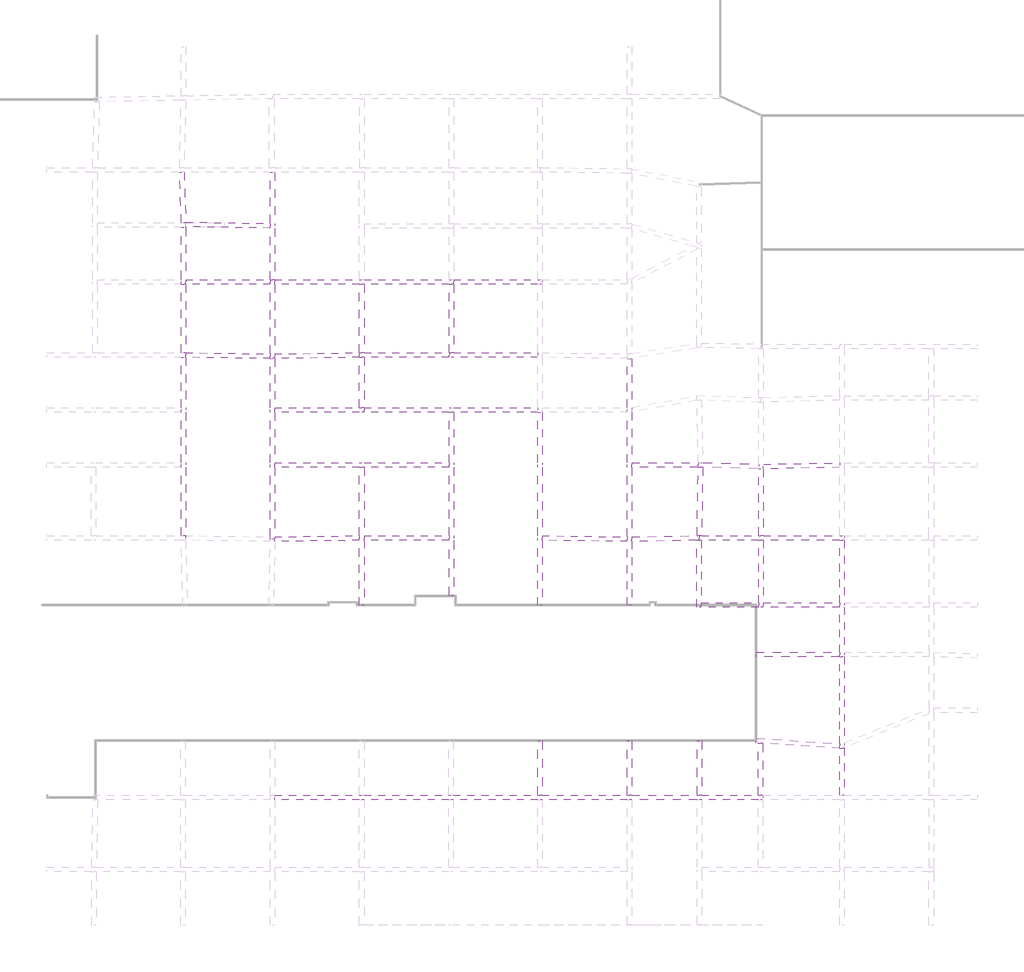
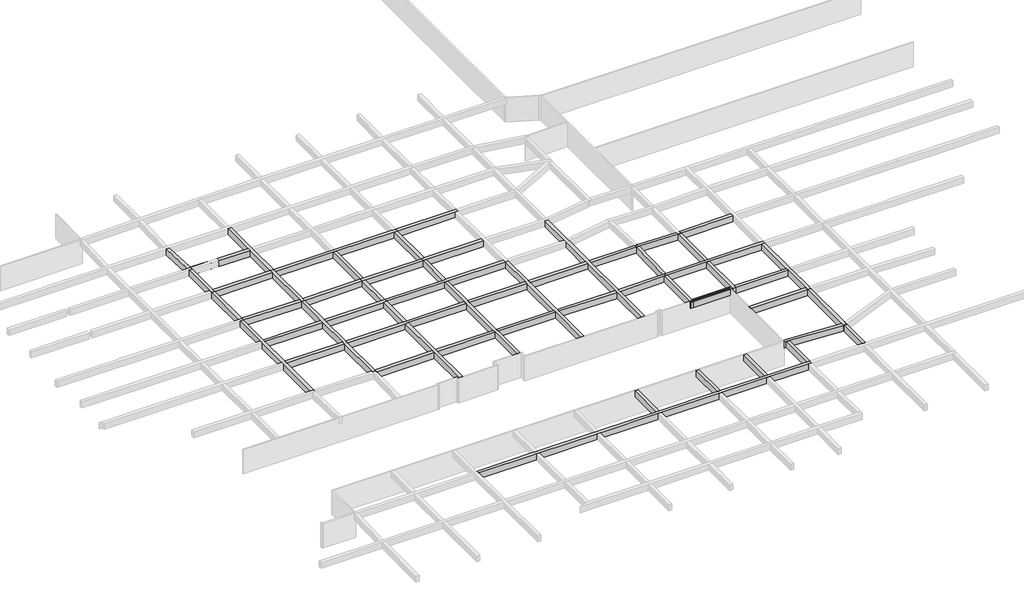
# One storey, part 14 of 20: 49 beams.
"""IFC4 building model written with IfcOpenShell, lengths in millimetres."""

from ifc_helpers import new_model, si_unit, frame, origin, place, context, project, spatial, polyline, outline, extrude, faceted_brep, element, save

model = new_model("IFC4")

# Units and contexts
model_context = context("Model", 3, world=origin())
ifc_project = project(units=[si_unit("LENGTHUNIT", "METRE", prefix="MILLI")], contexts=[model_context])

# Site, building, storey
site = spatial("IfcSite", under=ifc_project)
building = spatial("IfcBuilding", under=site)
storey = spatial("IfcBuildingStorey", under=building, Name="户型图", Elevation=0.0)

# Beams
placement = place(None, origin())
element("IfcBeam", 1, ObjectType="混凝土 - 矩形梁 : KL_beam", at=placement, inside=storey, context=model_context, shape_type="Brep", body=[
    faceted_brep([(183030.0, 66190.0, 3300.0), (183030.0, 66590.0, 3300.0), (182630.0, 66590.0, 3300.0), (177676.0, 66590.0, 3300.0), (177276.0, 66590.0, 3300.0), (171550.0, 66590.0, 3300.0), (171150.0, 66590.0, 3300.0), (163750.0, 66590.0, 3300.0), (163350.0, 66590.0, 3300.0), (155950.0, 66590.0, 3300.0), (155550.0, 66590.0, 3300.0), (148150.0, 66590.0, 3300.0), (147750.0, 66590.0, 3300.0), (140350.0, 66590.0, 3300.0), (140350.0, 66190.0, 3300.0), (147750.0, 66190.0, 3300.0), (148150.0, 66190.0, 3300.0), (155550.0, 66190.0, 3300.0), (155950.0, 66190.0, 3300.0), (163350.0, 66190.0, 3300.0), (163750.0, 66190.0, 3300.0), (171150.0, 66190.0, 3300.0), (171550.0, 66190.0, 3300.0), (177276.0, 66190.0, 3300.0), (177676.0, 66190.0, 3300.0), (182630.0, 66190.0, 3300.0), (183030.0, 66190.0, 2500.0), (140350.0, 66190.0, 2500.0), (147750.0, 66190.0, 2500.0), (148150.0, 66190.0, 2500.0), (155550.0, 66190.0, 2500.0), (155950.0, 66190.0, 2500.0), (163350.0, 66190.0, 2500.0), (163750.0, 66190.0, 2500.0), (171150.0, 66190.0, 2500.0), (171550.0, 66190.0, 2500.0), (177276.0, 66190.0, 2500.0), (177676.0, 66190.0, 2500.0), (182630.0, 66190.0, 2500.0), (183030.0, 66590.0, 2500.0), (140350.0, 66590.0, 2500.0), (147750.0, 66590.0, 2500.0), (148150.0, 66590.0, 2500.0), (155550.0, 66590.0, 2500.0), (155950.0, 66590.0, 2500.0), (163350.0, 66590.0, 2500.0), (163750.0, 66590.0, 2500.0), (171150.0, 66590.0, 2500.0), (171550.0, 66590.0, 2500.0), (177276.0, 66590.0, 2500.0), (177676.0, 66590.0, 2500.0), (182630.0, 66590.0, 2500.0)], [[[0, 1, 2, 3, 4, 5, 6, 7, 8, 9, 10, 11, 12, 13, 14, 15, 16, 17, 18, 19, 20, 21, 22, 23, 24, 25]], [[26, 0, 25, 24, 23, 22, 21, 20, 19, 18, 17, 16, 15, 14, 27, 28, 29, 30, 31, 32, 33, 34, 35, 36, 37, 38]], [[39, 26, 38, 37, 36, 35, 34, 33, 32, 31, 30, 29, 28, 27, 40, 41, 42, 43, 44, 45, 46, 47, 48, 49, 50, 51]], [[1, 39, 51, 50, 49, 48, 47, 46, 45, 44, 43, 42, 41, 40, 13, 12, 11, 10, 9, 8, 7, 6, 5, 4, 3, 2]], [[14, 13, 40, 27]], [[1, 0, 26, 39]]]),
])
element("IfcBeam", 2, ObjectType="混凝土 - 矩形梁 : KL_beam", at=placement, inside=storey, context=model_context, shape_type="Brep", body=[
    faceted_brep([(132150.0, 89290.0, 3300.0), (132544.9959727, 89290.0, 3300.0), (132550.0, 89092.5337107, 3300.0), (132550.0, 89287.4523333, 3300.0), (132550.0, 95290.0, 3300.0), (132550.0, 95690.0, 3300.0), (132550.0, 100089.0, 3300.0), (132550.0, 100489.0, 3300.0), (132550.0, 104885.6852836, 3300.0), (132550.0, 104889.0, 3300.0), (132150.0, 104889.0, 3300.0), (132150.0, 100489.0, 3300.0), (132150.0, 100089.0, 3300.0), (132150.0, 95690.0, 3300.0), (132150.0, 95290.0, 3300.0), (132150.0, 89290.0, 2500.0), (132150.0, 104889.0, 2500.0), (132150.0, 100489.0, 2500.0), (132150.0, 100089.0, 2500.0), (132150.0, 95690.0, 2500.0), (132150.0, 95290.0, 2500.0), (132544.9959727, 89290.0, 2500.0), (132550.0, 104889.0, 2500.0), (132550.0, 104885.6852836, 2500.0), (132550.0, 100489.0, 2500.0), (132550.0, 100089.0, 2500.0), (132550.0, 95690.0, 2500.0), (132550.0, 95290.0, 2500.0), (132550.0, 89287.4523333, 2500.0), (132550.0, 89092.5337107, 2500.0)], [[[0, 1, 2, 3, 4, 5, 6, 7, 8, 9, 10, 11, 12, 13, 14]], [[15, 0, 14, 13, 12, 11, 10, 16, 17, 18, 19, 20]], [[21, 15, 20, 19, 18, 17, 16, 22, 23, 24, 25, 26, 27, 28, 29]], [[2, 29, 28, 27, 26, 25, 24, 23, 22, 9, 8, 7, 6, 5, 4, 3]], [[21, 1, 0, 15]], [[1, 21, 29, 2]], [[10, 9, 22, 16]]]),
])
element("IfcBeam", 3, ObjectType="混凝土 - 矩形梁 : KL_beam", at=placement, inside=storey, context=model_context, shape_type="Brep", body=[
    faceted_brep([(132412.7389969, 121089.0, 3300.0), (132012.4951791, 121089.0, 3300.0), (132167.2640295, 116657.0, 3300.0), (132567.5078472, 116657.0, 3300.0), (132565.6031542, 116711.5432728, 3300.0), (132012.4951791, 121089.0, 2500.0), (132167.2640295, 116657.0, 2500.0), (132412.7389969, 121089.0, 2500.0), (132565.6031542, 116711.5432728, 2500.0), (132567.5078472, 116657.0, 2500.0)], [[[0, 1, 2, 3, 4]], [[1, 5, 6, 2]], [[5, 7, 8, 9, 6]], [[7, 0, 4, 3, 9, 8]], [[1, 0, 7, 5]], [[3, 2, 6, 9]]]),
])
element("IfcBeam", 4, ObjectType="混凝土 - 矩形梁 : KL_beam", at=placement, inside=storey, context=model_context, shape_type="Brep", body=[
    faceted_brep([(132172.3572995, 111289.0, 2500.0), (132172.3572995, 111289.0, 3300.0), (132172.3572995, 111689.0, 3300.0), (132172.3572995, 116257.0, 3300.0), (132172.3572995, 116257.0, 2500.0), (132172.3572995, 111689.0, 2500.0), (132572.3572995, 111289.0, 3300.0), (132572.3572995, 111289.0, 2500.0), (132572.3572995, 116257.0, 3300.0), (132572.3572995, 116257.0, 2500.0), (132572.3572995, 111689.0, 3300.0), (132572.3572995, 111689.0, 2500.0)], [[[0, 1, 2, 3, 4, 5]], [[6, 1, 0, 7]], [[8, 9, 4, 3]], [[1, 6, 10, 8, 3, 2]], [[7, 0, 5, 4, 9, 11]], [[6, 7, 11, 9, 8, 10]]]),
])
element("IfcBeam", 5, ObjectType="混凝土 - 矩形梁 : KL_beam", at=placement, inside=storey, context=model_context, shape_type="Brep", body=[
    faceted_brep([(132550.0, 104889.0, 3300.0), (132572.3572995, 104889.0, 3300.0), (132572.3572995, 105285.4331901, 3300.0), (132572.3572995, 111289.0, 3300.0), (132172.3572995, 111289.0, 3300.0), (132172.3572995, 105289.0, 3300.0), (132550.0, 105289.0, 3300.0), (132172.3572995, 105289.0, 2500.0), (132172.3572995, 111289.0, 2500.0), (132572.3572995, 104889.0, 2500.0), (132550.0, 104889.0, 2500.0), (132550.0, 105289.0, 2500.0), (132572.3572995, 111289.0, 2500.0), (132572.3572995, 105285.4331901, 2500.0)], [[[0, 1, 2, 3, 4, 5, 6]], [[7, 5, 4, 8]], [[9, 10, 11, 7, 8, 12, 13]], [[1, 9, 13, 12, 3, 2]], [[9, 1, 0, 10]], [[11, 6, 5, 7]], [[6, 11, 10, 0]], [[4, 3, 12, 8]]]),
])
element("IfcBeam", 6, ObjectType="混凝土 - 矩形梁 : KL_beam", at=placement, inside=storey, context=model_context, shape_type="Brep", body=[
    faceted_brep([(139950.0, 104791.5476667, 3300.0), (140350.0, 104791.5476667, 3300.0), (140350.0, 105191.5805384, 3300.0), (140350.0, 111289.0, 3300.0), (140350.0, 111689.0, 3300.0), (139950.0, 111689.0, 3300.0), (139950.0, 111289.0, 3300.0), (139950.0, 105191.5609646, 3300.0), (140350.0, 104791.5476667, 2500.0), (140350.0, 105191.5805384, 2500.0), (140350.0, 111289.0, 2500.0), (140350.0, 111689.0, 2500.0), (139950.0, 104791.5476667, 2500.0), (139950.0, 105191.5609646, 2500.0), (139950.0, 111289.0, 2500.0), (139950.0, 111689.0, 2500.0)], [[[0, 1, 2, 3, 4, 5, 6, 7]], [[1, 8, 9, 10, 11, 4, 3, 2]], [[8, 12, 13, 14, 15, 11, 10, 9]], [[12, 0, 7, 6, 5, 15, 14, 13]], [[5, 4, 11, 15]], [[0, 12, 8, 1]]]),
])
element("IfcBeam", 7, ObjectType="混凝土 - 矩形梁 : KL_beam", at=placement, inside=storey, context=model_context, shape_type="SweptSolid", body=[
    extrude(outline(polyline([(132572.3572995, 111289.0), (132572.3572995, 111689.0), (139950.0, 111689.0), (139950.0, 111289.0), (132572.3572995, 111289.0)])), frame((0.0, 0.0, 2500.0), z_axis=(0.0, 0.0, 1.0), x_axis=(1.0, 0.0, 0.0)), (0.0, 0.0, 1.0), 800.0),
])
element("IfcBeam", 8, ObjectType="混凝土 - 矩形梁 : KL_beam", at=placement, inside=storey, context=model_context, shape_type="Brep", body=[
    faceted_brep([(139950.0, 111689.0, 3300.0), (140350.0, 111689.0, 3300.0), (140350.0, 116189.0, 3300.0), (140350.0, 116589.0, 3300.0), (140350.0, 121089.0, 3300.0), (139950.0, 121089.0, 3300.0), (139950.0, 116592.2568622, 3300.0), (139950.0, 116192.2046763, 3300.0), (140350.0, 111689.0, 2500.0), (140350.0, 116189.0, 2500.0), (140350.0, 116589.0, 2500.0), (140350.0, 121089.0, 2500.0), (139950.0, 111689.0, 2500.0), (139950.0, 116192.2046763, 2500.0), (139950.0, 116592.2568622, 2500.0), (139950.0, 121089.0, 2500.0)], [[[0, 1, 2, 3, 4, 5, 6, 7]], [[1, 8, 9, 10, 11, 4, 3, 2]], [[8, 12, 13, 14, 15, 11, 10, 9]], [[12, 0, 7, 6, 5, 15, 14, 13]], [[1, 0, 12, 8]], [[5, 4, 11, 15]]]),
])
element("IfcBeam", 9, ObjectType="混凝土 - 矩形梁 : KL_beam", at=placement, inside=storey, context=model_context, shape_type="SweptSolid", body=[
    extrude(outline(polyline([(132572.3572995, 116518.1298566), (132572.3572995, 116657.0), (132567.5078472, 116657.0), (132565.6031542, 116711.5432728), (139950.0, 116592.2568622), (139950.0, 116192.2046763), (132579.5811694, 116311.2652881), (132572.3572995, 116518.1298566)])), frame((0.0, 0.0, 2500.0), z_axis=(0.0, 0.0, 1.0), x_axis=(1.0, 0.0, 0.0)), (0.0, 0.0, 1.0), 800.0),
])
element("IfcBeam", 10, ObjectType="混凝土 - 矩形梁 : KL_beam", at=placement, inside=storey, context=model_context, shape_type="Brep", body=[
    faceted_brep([(155979.0, 111289.0, 3300.0), (155979.0, 111689.0, 3300.0), (155579.0, 111689.0, 3300.0), (148150.0, 111689.0, 3300.0), (147750.0, 111689.0, 3300.0), (140350.0, 111689.0, 3300.0), (140350.0, 111289.0, 3300.0), (147750.0, 111289.0, 3300.0), (148150.0, 111289.0, 3300.0), (155579.0, 111289.0, 3300.0), (155979.0, 111289.0, 2500.0), (140350.0, 111289.0, 2500.0), (147750.0, 111289.0, 2500.0), (148150.0, 111289.0, 2500.0), (155579.0, 111289.0, 2500.0), (155979.0, 111689.0, 2500.0), (140350.0, 111689.0, 2500.0), (147750.0, 111689.0, 2500.0), (148150.0, 111689.0, 2500.0), (155579.0, 111689.0, 2500.0)], [[[0, 1, 2, 3, 4, 5, 6, 7, 8, 9]], [[10, 0, 9, 8, 7, 6, 11, 12, 13, 14]], [[15, 10, 14, 13, 12, 11, 16, 17, 18, 19]], [[1, 15, 19, 18, 17, 16, 5, 4, 3, 2]], [[6, 5, 16, 11]], [[1, 0, 10, 15]]]),
])
element("IfcBeam", 11, ObjectType="混凝土 - 矩形梁 : KL_beam", at=placement, inside=storey, context=model_context, shape_type="Brep", body=[
    faceted_brep([(163750.0, 111289.0, 3300.0), (163750.0, 111689.0, 3300.0), (163350.0, 111689.0, 3300.0), (155979.0, 111689.0, 3300.0), (155979.0, 111289.0, 3300.0), (163350.0, 111289.0, 3300.0), (163750.0, 111289.0, 2500.0), (155979.0, 111289.0, 2500.0), (163350.0, 111289.0, 2500.0), (163750.0, 111689.0, 2500.0), (155979.0, 111689.0, 2500.0), (163350.0, 111689.0, 2500.0)], [[[0, 1, 2, 3, 4, 5]], [[6, 0, 5, 4, 7, 8]], [[9, 6, 8, 7, 10, 11]], [[1, 9, 11, 10, 3, 2]], [[4, 3, 10, 7]], [[1, 0, 6, 9]]]),
])
element("IfcBeam", 12, ObjectType="混凝土 - 矩形梁 : KL_beam", at=placement, inside=storey, context=model_context, shape_type="Brep", body=[
    faceted_brep([(155579.0, 104889.0, 3300.0), (155579.0, 104889.0, 2500.0), (155979.0, 104889.0, 2500.0), (163350.0, 104889.0, 2500.0), (163350.0, 104889.0, 3300.0), (155979.0, 104889.0, 3300.0), (155579.0, 105289.0, 3300.0), (155579.0, 105289.0, 2500.0), (163350.0, 105289.0, 2500.0), (163350.0, 105289.0, 3300.0), (155979.0, 105289.0, 3300.0), (155979.0, 105289.0, 2500.0)], [[[0, 1, 2, 3, 4, 5]], [[0, 6, 7, 1]], [[4, 3, 8, 9]], [[6, 0, 5, 4, 9, 10]], [[7, 6, 10, 9, 8, 11]], [[1, 7, 11, 8, 3, 2]]]),
])
element("IfcBeam", 13, ObjectType="混凝土 - 矩形梁 : KL_beam", at=placement, inside=storey, context=model_context, shape_type="Brep", body=[
    faceted_brep([(147750.0, 105289.0, 3300.0), (147750.0, 105286.4523333, 3300.0), (147750.0, 104889.0, 3300.0), (148150.0, 104889.0, 3300.0), (155579.0, 104889.0, 3300.0), (155579.0, 105289.0, 3300.0), (148150.0, 105289.0, 3300.0), (147750.0, 105289.0, 2500.0), (155579.0, 105289.0, 2500.0), (148150.0, 105289.0, 2500.0), (147750.0, 104889.0, 2500.0), (147750.0, 105286.4523333, 2500.0), (155579.0, 104889.0, 2500.0), (148150.0, 104889.0, 2500.0)], [[[0, 1, 2, 3, 4, 5, 6]], [[7, 0, 6, 5, 8, 9]], [[10, 11, 7, 9, 8, 12, 13]], [[2, 10, 13, 12, 4, 3]], [[2, 1, 0, 7, 11, 10]], [[5, 4, 12, 8]]]),
])
element("IfcBeam", 14, ObjectType="混凝土 - 矩形梁 : KL_beam", at=placement, inside=storey, context=model_context, shape_type="SweptSolid", body=[
    extrude(outline(polyline([(148150.0, 105289.0), (147750.0, 105289.0), (147750.0, 111289.0), (148150.0, 111289.0), (148150.0, 105289.0)])), frame((0.0, 0.0, 2500.0), z_axis=(0.0, 0.0, 1.0), x_axis=(1.0, 0.0, 0.0)), (0.0, 0.0, 1.0), 800.0),
])
element("IfcBeam", 15, ObjectType="混凝土 - 矩形梁 : KL_beam", at=placement, inside=storey, context=model_context, shape_type="SweptSolid", body=[
    extrude(outline(polyline([(155579.0, 111289.0), (155979.0, 111289.0), (155979.0, 105289.0), (155579.0, 105289.0), (155579.0, 111289.0)])), frame((0.0, 0.0, 2500.0), z_axis=(0.0, 0.0, 1.0), x_axis=(1.0, 0.0, 0.0)), (0.0, 0.0, 1.0), 800.0),
])
element("IfcBeam", 16, ObjectType="混凝土 - 矩形梁 : KL_beam", at=placement, inside=storey, context=model_context, shape_type="Brep", body=[
    faceted_brep([(139950.0, 88991.7453736, 3300.0), (140350.0, 88988.2546264, 3300.0), (140350.0, 89187.4523333, 3300.0), (140350.0, 95290.0, 3300.0), (140350.0, 95690.0, 3300.0), (140350.0, 100089.0, 3300.0), (140350.0, 100489.0, 3300.0), (140350.0, 104791.5476667, 3300.0), (139950.0, 104786.4194616, 3300.0), (139950.0, 100489.0, 3300.0), (139950.0, 100089.0, 3300.0), (139950.0, 95690.0, 3300.0), (139950.0, 95290.0, 3300.0), (139950.0, 89192.5805384, 3300.0), (139950.0, 88991.7453736, 2500.0), (139950.0, 104786.4194616, 2500.0), (139950.0, 100489.0, 2500.0), (139950.0, 100089.0, 2500.0), (139950.0, 95690.0, 2500.0), (139950.0, 95290.0, 2500.0), (139950.0, 89192.5805384, 2500.0), (140350.0, 88988.2546264, 2500.0), (140350.0, 104791.5476667, 2500.0), (140350.0, 100489.0, 2500.0), (140350.0, 100089.0, 2500.0), (140350.0, 95690.0, 2500.0), (140350.0, 95290.0, 2500.0), (140350.0, 89187.4523333, 2500.0)], [[[0, 1, 2, 3, 4, 5, 6, 7, 8, 9, 10, 11, 12, 13]], [[14, 0, 13, 12, 11, 10, 9, 8, 15, 16, 17, 18, 19, 20]], [[21, 14, 20, 19, 18, 17, 16, 15, 22, 23, 24, 25, 26, 27]], [[1, 21, 27, 26, 25, 24, 23, 22, 7, 6, 5, 4, 3, 2]], [[1, 0, 14, 21]], [[8, 7, 22, 15]]]),
])
element("IfcBeam", 17, ObjectType="混凝土 - 矩形梁 : KL_beam", at=placement, inside=storey, context=model_context, shape_type="Brep", body=[
    faceted_brep([(140350.0, 88988.2546264, 3300.0), (140346.5831577, 88792.503861, 3300.0), (147750.0, 88887.4194616, 3300.0), (147750.0, 89287.4523333, 3300.0), (140350.0, 89192.5805384, 3300.0), (140350.0, 89187.4523333, 3300.0), (140346.5831577, 88792.503861, 2500.0), (147750.0, 88887.4194616, 2500.0), (140350.0, 88988.2546264, 2500.0), (140350.0, 89187.4523333, 2500.0), (140350.0, 89192.5805384, 2500.0), (147750.0, 89287.4523333, 2500.0)], [[[0, 1, 2, 3, 4, 5]], [[1, 6, 7, 2]], [[6, 8, 9, 10, 11, 7]], [[10, 4, 3, 11]], [[4, 10, 9, 8, 0, 5]], [[1, 0, 8, 6]], [[3, 2, 7, 11]]]),
])
element("IfcBeam", 18, ObjectType="混凝土 - 矩形梁 : KL_beam", at=placement, inside=storey, context=model_context, shape_type="Brep", body=[
    faceted_brep([(132550.0, 100489.0, 3300.0), (132550.0, 100089.0, 3300.0), (139950.0, 100089.0, 3300.0), (139950.0, 100489.0, 3300.0), (132550.0, 100089.0, 2500.0), (139950.0, 100089.0, 2500.0), (132550.0, 100489.0, 2500.0), (139950.0, 100489.0, 2500.0)], [[[0, 1, 2, 3]], [[1, 4, 5, 2]], [[4, 6, 7, 5]], [[6, 0, 3, 7]], [[1, 0, 6, 4]], [[3, 2, 5, 7]]]),
    faceted_brep([(140350.0, 100089.0, 3300.0), (140350.0, 100489.0, 3300.0), (140350.0, 100489.0, 2500.0), (140350.0, 100089.0, 2500.0), (148150.0, 100089.0, 3300.0), (148150.0, 100489.0, 3300.0), (147750.0, 100489.0, 3300.0), (147750.0, 100089.0, 3300.0), (148150.0, 100089.0, 2500.0), (147750.0, 100089.0, 2500.0), (148150.0, 100489.0, 2500.0), (147750.0, 100489.0, 2500.0)], [[[0, 1, 2, 3]], [[4, 5, 6, 1, 0, 7]], [[8, 4, 7, 0, 3, 9]], [[10, 8, 9, 3, 2, 11]], [[5, 10, 11, 2, 1, 6]], [[5, 4, 8, 10]]]),
])
element("IfcBeam", 19, ObjectType="混凝土 - 矩形梁 : KL_beam", at=placement, inside=storey, context=model_context, shape_type="Brep", body=[
    faceted_brep([(148150.0, 104889.0, 3300.0), (147750.0, 104889.0, 3300.0), (147750.0, 104886.4194616, 3300.0), (147750.0, 100489.0, 3300.0), (148150.0, 100489.0, 3300.0), (148150.0, 104889.0, 2500.0), (148150.0, 100489.0, 2500.0), (147750.0, 104889.0, 2500.0), (147750.0, 100489.0, 2500.0), (147750.0, 104886.4194616, 2500.0)], [[[0, 1, 2, 3, 4]], [[5, 0, 4, 6]], [[7, 5, 6, 8, 9]], [[1, 7, 9, 8, 3, 2]], [[1, 0, 5, 7]], [[4, 3, 8, 6]]]),
])
element("IfcBeam", 20, ObjectType="混凝土 - 矩形梁 : KL_beam", at=placement, inside=storey, context=model_context, shape_type="Brep", body=[
    faceted_brep([(139950.0, 104786.4194616, 3300.0), (139950.0, 104786.4194616, 2500.0), (140350.0, 104791.5476667, 2500.0), (147750.0, 104886.4194616, 2500.0), (147750.0, 104886.4194616, 3300.0), (140350.0, 104791.5476667, 3300.0), (139950.0, 104791.5476667, 3300.0), (139950.0, 104791.5476667, 2500.0), (140350.0, 105191.5805384, 3300.0), (140350.0, 105191.5805384, 2500.0), (147750.0, 104889.0, 2500.0), (147750.0, 105286.4523333, 2500.0), (147750.0, 105286.4523333, 3300.0), (147750.0, 104889.0, 3300.0)], [[[0, 1, 2, 3, 4, 5]], [[1, 0, 6, 7]], [[2, 5, 8, 9]], [[5, 2, 7, 6]], [[6, 0, 5]], [[1, 7, 2]], [[4, 3, 10, 11, 12, 13]], [[8, 5, 4, 13, 12]], [[9, 8, 12, 11]], [[2, 9, 11, 10, 3]]]),
])
element("IfcBeam", 21, ObjectType="混凝土 - 矩形梁 : KL_beam", at=placement, inside=storey, context=model_context, shape_type="SweptSolid", body=[
    extrude(outline(polyline([(139950.0, 105191.5609646), (139950.0, 104791.5285865), (132550.0, 104885.6852836), (132550.0, 104889.0), (132572.3572995, 104889.0), (132572.3572995, 105285.4331901), (139950.0, 105191.5609646)])), frame((0.0, 0.0, 2500.0), z_axis=(0.0, 0.0, 1.0), x_axis=(1.0, 0.0, 0.0)), (0.0, 0.0, 1.0), 800.0),
])
element("IfcBeam", 22, ObjectType="混凝土 - 矩形梁 : KL_beam", at=placement, inside=storey, context=model_context, shape_type="Brep", body=[
    faceted_brep([(163350.0, 100089.0, 3300.0), (163350.0, 100489.0, 3300.0), (155979.0, 100489.0, 3300.0), (155579.0, 100489.0, 3300.0), (148150.0, 100489.0, 3300.0), (148150.0, 100089.0, 3300.0), (155579.0, 100089.0, 3300.0), (155979.0, 100089.0, 3300.0), (163350.0, 100089.0, 2500.0), (148150.0, 100089.0, 2500.0), (155579.0, 100089.0, 2500.0), (155979.0, 100089.0, 2500.0), (163350.0, 100489.0, 2500.0), (148150.0, 100489.0, 2500.0), (155579.0, 100489.0, 2500.0), (155979.0, 100489.0, 2500.0)], [[[0, 1, 2, 3, 4, 5, 6, 7]], [[8, 0, 7, 6, 5, 9, 10, 11]], [[12, 8, 11, 10, 9, 13, 14, 15]], [[1, 12, 15, 14, 13, 4, 3, 2]], [[1, 0, 8, 12]], [[5, 4, 13, 9]]]),
])
element("IfcBeam", 23, ObjectType="混凝土 - 矩形梁 : KL_beam", at=placement, inside=storey, context=model_context, shape_type="Brep", body=[
    faceted_brep([(171550.0, 83220.427457, 3300.0), (171150.0, 83220.427457, 3300.0), (171150.0, 83220.427457, 2500.0), (171550.0, 83220.427457, 2500.0), (171550.0, 88788.7316812, 3300.0), (171550.0, 89188.7926124, 3300.0), (171550.0, 95290.0, 3300.0), (171550.0, 95690.0, 3300.0), (171550.0, 100120.9198866, 3300.0), (171550.0, 100526.9817528, 3300.0), (171550.0, 104783.1926823, 3300.0), (171364.4255325, 104785.6466688, 3300.0), (171212.573786, 104761.5957149, 3300.0), (171208.4377833, 104787.7094085, 3300.0), (171150.0, 104788.4821739, 3300.0), (171150.0, 100489.0, 3300.0), (171150.0, 100089.0, 3300.0), (171150.0, 95690.0, 3300.0), (171150.0, 95290.0, 3300.0), (171150.0, 89187.9745164, 3300.0), (171150.0, 88787.9384623, 3300.0), (171150.0, 104788.4821739, 2500.0), (171150.0, 100489.0, 2500.0), (171150.0, 100089.0, 2500.0), (171150.0, 95690.0, 2500.0), (171150.0, 95290.0, 2500.0), (171150.0, 89187.9745164, 2500.0), (171150.0, 88787.9384623, 2500.0), (171208.4377833, 104787.7094085, 2500.0), (171212.573786, 104761.5957149, 2500.0), (171364.4255325, 104785.6466688, 2500.0), (171550.0, 104783.1926823, 2500.0), (171550.0, 100526.9817528, 2500.0), (171550.0, 100120.9198866, 2500.0), (171550.0, 95690.0, 2500.0), (171550.0, 95290.0, 2500.0), (171550.0, 89188.7926124, 2500.0), (171550.0, 88788.7316812, 2500.0)], [[[0, 1, 2, 3]], [[1, 0, 4, 5, 6, 7, 8, 9, 10, 11, 12, 13, 14, 15, 16, 17, 18, 19, 20]], [[2, 1, 20, 19, 18, 17, 16, 15, 14, 21, 22, 23, 24, 25, 26, 27]], [[3, 2, 27, 26, 25, 24, 23, 22, 21, 28, 29, 30, 31, 32, 33, 34, 35, 36, 37]], [[0, 3, 37, 36, 35, 34, 33, 32, 31, 10, 9, 8, 7, 6, 5, 4]], [[29, 12, 11, 30]], [[12, 29, 28, 13]], [[14, 13, 28, 21]], [[11, 10, 31, 30]]]),
])
element("IfcBeam", 24, ObjectType="混凝土 - 矩形梁 : KL_beam", at=placement, inside=storey, context=model_context, shape_type="Brep", body=[
    faceted_brep([(163750.0, 83220.0, 3300.0), (163350.0, 83220.0, 3300.0), (163350.0, 83220.0, 2500.0), (163750.0, 83220.0, 2500.0), (163750.0, 88887.2966174, 3300.0), (163750.0, 89287.3326715, 3300.0), (163750.0, 95290.0, 3300.0), (163750.0, 95690.0, 3300.0), (163750.0, 100089.0, 3300.0), (163350.0, 100089.0, 3300.0), (163350.0, 95690.0, 3300.0), (163350.0, 95290.0, 3300.0), (163350.0, 89290.0, 3300.0), (163350.0, 88890.0, 3300.0), (163350.0, 100089.0, 2500.0), (163350.0, 95690.0, 2500.0), (163350.0, 95290.0, 2500.0), (163350.0, 89290.0, 2500.0), (163350.0, 88890.0, 2500.0), (163750.0, 100089.0, 2500.0), (163750.0, 95690.0, 2500.0), (163750.0, 95290.0, 2500.0), (163750.0, 89287.3326715, 2500.0), (163750.0, 88887.2966174, 2500.0)], [[[0, 1, 2, 3]], [[1, 0, 4, 5, 6, 7, 8, 9, 10, 11, 12, 13]], [[2, 1, 13, 12, 11, 10, 9, 14, 15, 16, 17, 18]], [[3, 2, 18, 17, 16, 15, 14, 19, 20, 21, 22, 23]], [[0, 3, 23, 22, 21, 20, 19, 8, 7, 6, 5, 4]], [[9, 8, 19, 14]]]),
])
element("IfcBeam", 25, ObjectType="混凝土 - 矩形梁 : KL_beam", at=placement, inside=storey, context=model_context, shape_type="Brep", body=[
    faceted_brep([(155979.0, 84020.0, 3300.0), (155579.0, 84020.0, 3300.0), (155579.0, 84020.0, 2500.0), (155979.0, 84020.0, 2500.0), (155979.0, 88890.0, 3300.0), (155979.0, 89290.0, 3300.0), (155979.0, 95290.0, 3300.0), (155979.0, 95690.0, 3300.0), (155979.0, 100089.0, 3300.0), (155579.0, 100089.0, 3300.0), (155579.0, 95690.0, 3300.0), (155579.0, 95290.0, 3300.0), (155579.0, 89290.0, 3300.0), (155579.0, 88890.0, 3300.0), (155579.0, 100089.0, 2500.0), (155579.0, 95690.0, 2500.0), (155579.0, 95290.0, 2500.0), (155579.0, 89290.0, 2500.0), (155579.0, 88890.0, 2500.0), (155979.0, 100089.0, 2500.0), (155979.0, 95690.0, 2500.0), (155979.0, 95290.0, 2500.0), (155979.0, 89290.0, 2500.0), (155979.0, 88890.0, 2500.0)], [[[0, 1, 2, 3]], [[1, 0, 4, 5, 6, 7, 8, 9, 10, 11, 12, 13]], [[2, 1, 13, 12, 11, 10, 9, 14, 15, 16, 17, 18]], [[3, 2, 18, 17, 16, 15, 14, 19, 20, 21, 22, 23]], [[0, 3, 23, 22, 21, 20, 19, 8, 7, 6, 5, 4]], [[9, 8, 19, 14]]]),
    faceted_brep([(155579.0, 104889.0, 3300.0), (155979.0, 104889.0, 3300.0), (155979.0, 104889.0, 2500.0), (155579.0, 104889.0, 2500.0), (155979.0, 100489.0, 3300.0), (155579.0, 100489.0, 3300.0), (155579.0, 100489.0, 2500.0), (155979.0, 100489.0, 2500.0)], [[[0, 1, 2, 3]], [[4, 5, 6, 7]], [[1, 0, 5, 4]], [[0, 3, 6, 5]], [[3, 2, 7, 6]], [[2, 1, 4, 7]]]),
])
element("IfcBeam", 26, ObjectType="混凝土 - 矩形梁 : KL_beam", at=placement, inside=storey, context=model_context, shape_type="Brep", body=[
    faceted_brep([(132550.0, 95690.0, 3300.0), (132550.0, 95290.0, 3300.0), (139950.0, 95290.0, 3300.0), (139950.0, 95690.0, 3300.0), (132550.0, 95290.0, 2500.0), (139950.0, 95290.0, 2500.0), (132550.0, 95690.0, 2500.0), (139950.0, 95690.0, 2500.0)], [[[0, 1, 2, 3]], [[1, 4, 5, 2]], [[4, 6, 7, 5]], [[6, 0, 3, 7]], [[1, 0, 6, 4]], [[3, 2, 5, 7]]]),
    faceted_brep([(171150.0, 95690.0, 3300.0), (171150.0, 95290.0, 3300.0), (171150.0, 95290.0, 2500.0), (171150.0, 95690.0, 2500.0), (163750.0, 95690.0, 3300.0), (163750.0, 95290.0, 3300.0), (163750.0, 95290.0, 2500.0), (163750.0, 95690.0, 2500.0)], [[[0, 1, 2, 3]], [[1, 0, 4, 5]], [[2, 1, 5, 6]], [[3, 2, 6, 7]], [[0, 3, 7, 4]], [[5, 4, 7, 6]]]),
    faceted_brep([(140350.0, 95290.0, 3300.0), (140350.0, 95690.0, 3300.0), (140350.0, 95690.0, 2500.0), (140350.0, 95290.0, 2500.0), (155579.0, 95690.0, 3300.0), (155579.0, 95290.0, 3300.0), (155579.0, 95290.0, 2500.0), (155579.0, 95690.0, 2500.0), (147750.0, 95290.0, 3300.0), (148150.0, 95290.0, 3300.0), (148150.0, 95690.0, 3300.0), (147750.0, 95690.0, 3300.0), (147750.0, 95290.0, 2500.0), (148150.0, 95290.0, 2500.0), (147750.0, 95690.0, 2500.0), (148150.0, 95690.0, 2500.0)], [[[0, 1, 2, 3]], [[4, 5, 6, 7]], [[1, 0, 8, 9, 5, 4, 10, 11]], [[0, 3, 12, 13, 6, 5, 9, 8]], [[3, 2, 14, 15, 7, 6, 13, 12]], [[2, 1, 11, 10, 4, 7, 15, 14]]]),
    faceted_brep([(163350.0, 95690.0, 3300.0), (163350.0, 95290.0, 3300.0), (163350.0, 95290.0, 2500.0), (163350.0, 95690.0, 2500.0), (155979.0, 95690.0, 3300.0), (155979.0, 95290.0, 3300.0), (155979.0, 95290.0, 2500.0), (155979.0, 95690.0, 2500.0)], [[[0, 1, 2, 3]], [[1, 0, 4, 5]], [[2, 1, 5, 6]], [[3, 2, 6, 7]], [[0, 3, 7, 4]], [[5, 4, 7, 6]]]),
])
element("IfcBeam", 27, ObjectType="混凝土 - 矩形梁 : KL_beam", at=placement, inside=storey, context=model_context, shape_type="Brep", body=[
    faceted_brep([(148150.0, 83220.0, 3300.0), (147750.0, 83220.0, 3300.0), (147750.0, 83220.0, 2500.0), (148150.0, 83220.0, 2500.0), (148150.0, 88890.0, 3300.0), (148150.0, 89290.0, 3300.0), (148150.0, 95290.0, 3300.0), (147750.0, 95290.0, 3300.0), (147750.0, 89287.4523333, 3300.0), (147750.0, 88887.4194616, 3300.0), (147750.0, 95290.0, 2500.0), (147750.0, 89287.4523333, 2500.0), (147750.0, 88887.4194616, 2500.0), (148150.0, 95290.0, 2500.0), (148150.0, 89290.0, 2500.0), (148150.0, 88890.0, 2500.0)], [[[0, 1, 2, 3]], [[1, 0, 4, 5, 6, 7, 8, 9]], [[2, 1, 9, 8, 7, 10, 11, 12]], [[3, 2, 12, 11, 10, 13, 14, 15]], [[0, 3, 15, 14, 13, 6, 5, 4]], [[7, 6, 13, 10]]]),
    faceted_brep([(147750.0, 100089.0, 3300.0), (148150.0, 100089.0, 3300.0), (148150.0, 100089.0, 2500.0), (147750.0, 100089.0, 2500.0), (148150.0, 95690.0, 3300.0), (147750.0, 95690.0, 3300.0), (147750.0, 95690.0, 2500.0), (148150.0, 95690.0, 2500.0)], [[[0, 1, 2, 3]], [[4, 5, 6, 7]], [[1, 0, 5, 4]], [[0, 3, 6, 5]], [[3, 2, 7, 6]], [[2, 1, 4, 7]]]),
])
element("IfcBeam", 28, ObjectType="混凝土 - 矩形梁 : KL_beam", at=placement, inside=storey, context=model_context, shape_type="SweptSolid", body=[
    extrude(outline(polyline([(148150.0, 88890.0), (148150.0, 89290.0), (155579.0, 89290.0), (155579.0, 88890.0), (148150.0, 88890.0)])), frame((0.0, 0.0, 2500.0), z_axis=(0.0, 0.0, 1.0), x_axis=(1.0, 0.0, 0.0)), (0.0, 0.0, 1.0), 800.0),
    extrude(outline(polyline([(163350.0, 89290.0), (163350.0, 88890.0), (155979.0, 88890.0), (155979.0, 89290.0), (163350.0, 89290.0)])), frame((0.0, 0.0, 2500.0), z_axis=(0.0, 0.0, 1.0), x_axis=(1.0, 0.0, 0.0)), (0.0, 0.0, 1.0), 800.0),
])
element("IfcBeam", 29, ObjectType="混凝土 - 矩形梁 : KL_beam", at=placement, inside=storey, context=model_context, shape_type="SweptSolid", body=[
    extrude(outline(polyline([(171150.0, 89187.9745164), (171150.0, 88787.9384623), (163750.0, 88887.2966174), (163750.0, 89287.3326715), (171150.0, 89187.9745164)])), frame((0.0, 0.0, 2500.0), z_axis=(0.0, 0.0, 1.0), x_axis=(1.0, 0.0, 0.0)), (0.0, 0.0, 1.0), 800.0),
])
element("IfcBeam", 30, ObjectType="混凝土 - 矩形梁 : KL_beam", at=placement, inside=storey, context=model_context, shape_type="Brep", body=[
    faceted_brep([(177451.7795069, 88891.7476257, 3300.0), (177448.2887598, 89291.7476257, 3300.0), (177266.7233175, 89288.5783891, 3300.0), (171550.0, 89188.7926124, 3300.0), (171550.0, 88788.7316812, 3300.0), (177250.0341333, 88888.2261471, 3300.0), (177451.7795069, 88891.7476257, 2500.0), (171550.0, 88788.7316812, 2500.0), (177250.0341333, 88888.2261471, 2500.0), (177448.2887598, 89291.7476257, 2500.0), (171550.0, 89188.7926124, 2500.0), (177266.7233175, 89288.5783891, 2500.0)], [[[0, 1, 2, 3, 4, 5]], [[6, 0, 5, 4, 7, 8]], [[9, 6, 8, 7, 10, 11]], [[1, 9, 11, 10, 3, 2]], [[4, 3, 10, 7]], [[1, 0, 6, 9]]]),
])
element("IfcBeam", 31, ObjectType="混凝土 - 矩形梁 : KL_beam", at=placement, inside=storey, context=model_context, shape_type="Brep", body=[
    faceted_brep([(177448.2887598, 89291.7476257, 3300.0), (177451.7795069, 88891.7476257, 3300.0), (177650.0341333, 88891.7476257, 3300.0), (182646.7104659, 88891.7476257, 3300.0), (183046.7104659, 88891.7476257, 3300.0), (189750.0341333, 88891.7476257, 3300.0), (190150.0341333, 88891.7476257, 3300.0), (190150.0341333, 89291.7476257, 3300.0), (189750.0341333, 89291.7476257, 3300.0), (183046.7104659, 89291.7476257, 3300.0), (182646.7104659, 89291.7476257, 3300.0), (177666.839568, 89291.7476257, 3300.0), (177650.0341333, 89291.7476257, 3300.0), (177451.7795069, 88891.7476257, 2500.0), (177650.0341333, 88891.7476257, 2500.0), (182646.7104659, 88891.7476257, 2500.0), (183046.7104659, 88891.7476257, 2500.0), (189750.0341333, 88891.7476257, 2500.0), (190150.0341333, 88891.7476257, 2500.0), (177448.2887598, 89291.7476257, 2500.0), (177650.0341333, 89291.7476257, 2500.0), (177666.839568, 89291.7476257, 2500.0), (182646.7104659, 89291.7476257, 2500.0), (183046.7104659, 89291.7476257, 2500.0), (189750.0341333, 89291.7476257, 2500.0), (190150.0341333, 89291.7476257, 2500.0)], [[[0, 1, 2, 3, 4, 5, 6, 7, 8, 9, 10, 11, 12]], [[1, 13, 14, 15, 16, 17, 18, 6, 5, 4, 3, 2]], [[13, 19, 20, 21, 22, 23, 24, 25, 18, 17, 16, 15, 14]], [[19, 0, 12, 11, 10, 9, 8, 7, 25, 24, 23, 22, 21, 20]], [[0, 19, 13, 1]], [[7, 6, 18, 25]]]),
])
element("IfcBeam", 32, ObjectType="混凝土 - 矩形梁 : KL_beam", at=placement, inside=storey, context=model_context, shape_type="SweptSolid", body=[
    extrude(outline(polyline([(183046.7104659, 89291.7476257), (182646.7104659, 89291.7476257), (182646.7104659, 95145.5428717), (183046.7104659, 95134.1560933), (183046.7104659, 89291.7476257)])), frame((0.0, 0.0, 2500.0), z_axis=(0.0, 0.0, 1.0), x_axis=(1.0, 0.0, 0.0)), (0.0, 0.0, 1.0), 800.0),
])
element("IfcBeam", 33, ObjectType="混凝土 - 矩形梁 : KL_beam", at=placement, inside=storey, context=model_context, shape_type="Brep", body=[
    faceted_brep([(183046.7104659, 95134.1560933, 3300.0), (183046.7104659, 95145.5428717, 3300.0), (182646.7104659, 95145.5428717, 3300.0), (183046.7104659, 95134.1560933, 2500.0), (177771.4404287, 95284.3269206, 3300.0), (177371.5781859, 95295.7097775, 3300.0), (177371.5781859, 95295.7097775, 2500.0), (177771.4404287, 95284.3269206, 2500.0), (182646.7104659, 95145.5428717, 2500.0), (183046.7104659, 95145.5428717, 2500.0), (177382.9603534, 95695.5478025, 2500.0), (177382.9603534, 95695.5478025, 3300.0), (177577.8461181, 95690.0, 3300.0), (177770.8999723, 95684.5043464, 3300.0), (182646.7104659, 95545.7049123, 3300.0), (182646.7104659, 95545.7049123, 2500.0), (177770.8999723, 95684.5043464, 2500.0), (177577.8461181, 95690.0, 2500.0)], [[[0, 1, 2]], [[3, 0, 2, 4, 5, 6, 7, 8]], [[9, 3, 8]], [[10, 11, 12, 13, 14, 15, 16, 17]], [[0, 3, 9, 1]], [[2, 8, 15, 14]], [[8, 2, 1, 9]], [[11, 5, 4, 2, 14, 13, 12]], [[6, 10, 17, 16, 15, 8, 7]], [[11, 10, 6, 5]]]),
])
element("IfcBeam", 34, ObjectType="混凝土 - 矩形梁 : KL_beam", at=placement, inside=storey, context=model_context, shape_type="Brep", body=[
    faceted_brep([(183046.7104659, 95543.4519814, 2500.0), (183046.7104659, 95543.4519814, 3300.0), (189750.0341333, 95660.4589312, 3300.0), (189750.0341333, 95660.4589312, 2500.0), (183046.7104659, 95145.5428717, 2500.0), (183046.7104659, 95143.3910502, 2500.0), (183046.7104659, 95143.3910502, 3300.0), (183046.7104659, 95145.5428717, 3300.0), (189750.0341333, 95260.398, 3300.0), (189750.0341333, 95260.398, 2500.0)], [[[0, 1, 2, 3]], [[1, 0, 4, 5, 6, 7]], [[1, 7, 6, 8, 2]], [[6, 5, 9, 8]], [[5, 4, 0, 3, 9]], [[3, 2, 8, 9]]]),
])
element("IfcBeam", 35, ObjectType="混凝土 - 矩形梁 : KL_beam", at=placement, inside=storey, context=model_context, shape_type="Brep", body=[
    faceted_brep([(177650.0341333, 89294.140534, 3300.0), (177585.3783875, 89294.140534, 3300.0), (177448.2887598, 89291.7476257, 3300.0), (177650.0341333, 89291.7476257, 3300.0), (177650.0341333, 89294.140534, 2500.0), (177650.0341333, 89291.7476257, 2500.0), (177585.3783875, 89294.140534, 2500.0), (177448.2887598, 89291.7476257, 2500.0)], [[[0, 1, 2, 3]], [[4, 0, 3, 5]], [[0, 4, 6, 1]], [[1, 6, 7, 2]], [[3, 2, 7, 5]], [[6, 4, 5, 7]]]),
    faceted_brep([(177250.0341333, 88888.2261471, 3300.0), (177250.0341333, 88888.2261471, 2500.0), (177250.0341333, 83020.0, 2500.0), (177250.0341333, 83020.0, 3300.0), (177451.7795069, 88891.7476257, 2500.0), (177650.0341333, 88891.7476257, 2500.0), (177650.0341333, 83420.0, 2500.0), (177650.0341333, 83020.0, 2500.0), (177451.7795069, 88891.7476257, 3300.0), (177650.0341333, 88891.7476257, 3300.0), (177650.0341333, 83020.0, 3300.0), (177650.0341333, 83420.0, 3300.0)], [[[0, 1, 2, 3]], [[1, 4, 5, 6, 7, 2]], [[0, 8, 4, 1]], [[8, 9, 5, 4]], [[8, 0, 3, 10, 11, 9]], [[10, 7, 6, 5, 9, 11]], [[10, 3, 2, 7]]]),
])
element("IfcBeam", 36, ObjectType="混凝土 - 矩形梁 : KL_beam", at=placement, inside=storey, context=model_context, shape_type="Brep", body=[
    faceted_brep([(177771.4404287, 95284.3269206, 3300.0), (177371.5781859, 95295.7097775, 3300.0), (177371.4785214, 95290.0, 3300.0), (177266.7233175, 89288.5783891, 3300.0), (177448.2887598, 89291.7476257, 3300.0), (177585.3783875, 89294.140534, 3300.0), (177650.0341333, 89294.140534, 3300.0), (177650.0341333, 89291.7476257, 3300.0), (177666.839568, 89291.7476257, 3300.0), (177378.5595713, 95695.6730794, 3300.0), (177378.5595713, 95695.6730794, 2500.0), (177378.4605474, 95690.0, 2500.0), (177371.5781859, 95295.7097775, 2500.0), (177371.4785214, 95290.0, 2500.0), (177266.7233175, 89288.5783891, 2500.0), (177378.4605474, 95690.0, 3300.0), (177382.9603534, 95695.5478025, 2500.0), (177771.4404287, 95284.3269206, 2500.0), (177666.839568, 89291.7476257, 2500.0), (177382.9603534, 95695.5478025, 3300.0), (177650.0341333, 89291.7476257, 2500.0), (177650.0341333, 89294.140534, 2500.0), (177585.3783875, 89294.140534, 2500.0), (177448.2887598, 89291.7476257, 2500.0)], [[[0, 1, 2, 3, 4, 5, 6, 7, 8]], [[9, 10, 11, 12, 13, 14, 3, 2, 1, 15]], [[10, 16, 12, 11]], [[17, 0, 8, 18]], [[10, 9, 19, 16]], [[12, 1, 0, 17]], [[1, 12, 16, 19]], [[19, 9, 15, 1]], [[12, 17, 18, 20, 21, 22, 23, 14, 13]], [[18, 8, 7, 20]], [[3, 14, 23, 22, 5, 4]], [[6, 21, 20, 7]], [[21, 6, 5, 22]]]),
])
element("IfcBeam", 37, ObjectType="混凝土 - 矩形梁 : KL_beam", at=placement, inside=storey, context=model_context, shape_type="Brep", body=[
    faceted_brep([(177770.7828441, 95690.0, 3300.0), (177577.8461181, 95690.0, 3300.0), (177770.8999723, 95684.5043464, 3300.0), (177577.8461181, 95690.0, 2500.0), (177770.7828441, 95690.0, 2500.0), (177770.8999723, 95684.5043464, 2500.0)], [[[0, 1, 2]], [[3, 4, 5]], [[1, 0, 4, 3]], [[2, 1, 3, 5]], [[4, 0, 2, 5]]]),
    faceted_brep([(177371.4785214, 95290.0, 2500.0), (177371.4785214, 95290.0, 3300.0), (171550.0, 95290.0, 3300.0), (171550.0, 95290.0, 2500.0), (177371.5781859, 95295.7097775, 2500.0), (177378.4605474, 95690.0, 2500.0), (177378.4605474, 95690.0, 3300.0), (177371.5781859, 95295.7097775, 3300.0), (171550.0, 95690.0, 3300.0), (171550.0, 95690.0, 2500.0), (177370.6920067, 95690.0, 3300.0), (177370.6920067, 95690.0, 2500.0)], [[[0, 1, 2, 3]], [[1, 0, 4, 5, 6, 7]], [[3, 2, 8, 9]], [[1, 7, 6, 10, 8, 2]], [[4, 0, 3, 9, 11, 5]], [[6, 5, 11, 9, 8, 10]]]),
])
element("IfcBeam", 38, ObjectType="混凝土 - 矩形梁 : KL_beam", at=placement, inside=storey, context=model_context, shape_type="Brep", body=[
    faceted_brep([(189750.0341333, 78691.7476257, 3300.0), (190150.0341333, 78691.7476257, 3300.0), (190150.0341333, 79091.7476257, 3300.0), (190150.0341333, 83020.0, 3300.0), (190150.0341333, 83420.0, 3300.0), (190150.0341333, 88891.7476257, 3300.0), (189750.0341333, 88891.7476257, 3300.0), (189750.0341333, 83420.0, 3300.0), (189750.0341333, 83020.0, 3300.0), (189750.0341333, 79091.7476257, 3300.0), (189750.0341333, 78691.7476257, 2500.0), (189750.0341333, 88891.7476257, 2500.0), (189750.0341333, 83420.0, 2500.0), (189750.0341333, 83020.0, 2500.0), (189750.0341333, 79091.7476257, 2500.0), (190150.0341333, 78691.7476257, 2500.0), (190150.0341333, 88891.7476257, 2500.0), (190150.0341333, 83420.0, 2500.0), (190150.0341333, 83020.0, 2500.0), (190150.0341333, 79091.7476257, 2500.0)], [[[0, 1, 2, 3, 4, 5, 6, 7, 8, 9]], [[10, 0, 9, 8, 7, 6, 11, 12, 13, 14]], [[15, 10, 14, 13, 12, 11, 16, 17, 18, 19]], [[1, 15, 19, 18, 17, 16, 5, 4, 3, 2]], [[6, 5, 16, 11]], [[1, 0, 10, 15]]]),
])
element("IfcBeam", 39, ObjectType="混凝土 - 矩形梁 : KL_beam", at=placement, inside=storey, context=model_context, shape_type="Brep", body=[
    faceted_brep([(189750.0341333, 70704.0725066, 3300.0), (190150.0341333, 70704.0725066, 3300.0), (190150.0341333, 71187.6272479, 3300.0), (190150.0341333, 78691.7476257, 3300.0), (189750.0341333, 78691.7476257, 3300.0), (189750.0341333, 71104.8818984, 3300.0), (189750.0341333, 70704.0725066, 2500.0), (189750.0341333, 78691.7476257, 2500.0), (189750.0341333, 71104.8818984, 2500.0), (190150.0341333, 70704.0725066, 2500.0), (190150.0341333, 78691.7476257, 2500.0), (190150.0341333, 71187.6272479, 2500.0)], [[[0, 1, 2, 3, 4, 5]], [[6, 0, 5, 4, 7, 8]], [[9, 6, 8, 7, 10, 11]], [[1, 9, 11, 10, 3, 2]], [[4, 3, 10, 7]], [[1, 0, 6, 9]]]),
])
element("IfcBeam", 40, ObjectType="混凝土 - 矩形梁 : KL_beam", at=placement, inside=storey, context=model_context, shape_type="SweptSolid", body=[
    extrude(outline(polyline([(182436.0170667, 78691.7476257), (182436.0170667, 79091.7476257), (189750.0341333, 79091.7476257), (189750.0341333, 78691.7476257), (182436.0170667, 78691.7476257)])), frame((0.0, 0.0, 2500.0), z_axis=(0.0, 0.0, 1.0), x_axis=(1.0, 0.0, 0.0)), (0.0, 0.0, 1.0), 800.0),
])
element("IfcBeam", 41, ObjectType="混凝土 - 矩形梁 : KL_beam", at=placement, inside=storey, context=model_context, shape_type="Brep", body=[
    faceted_brep([(182646.7104659, 83020.0, 3300.0), (183046.7104659, 83020.0, 3300.0), (183046.7104659, 83420.0, 3300.0), (183046.7104659, 88891.7476257, 3300.0), (182646.7104659, 88891.7476257, 3300.0), (182646.7104659, 83420.0, 3300.0), (182646.7104659, 83020.0, 2500.0), (182646.7104659, 88891.7476257, 2500.0), (182646.7104659, 83420.0, 2500.0), (183046.7104659, 83020.0, 2500.0), (183046.7104659, 88891.7476257, 2500.0), (183046.7104659, 83420.0, 2500.0)], [[[0, 1, 2, 3, 4, 5]], [[6, 0, 5, 4, 7, 8]], [[9, 6, 8, 7, 10, 11]], [[1, 9, 11, 10, 3, 2]], [[4, 3, 10, 7]], [[1, 0, 6, 9]]]),
])
element("IfcBeam", 42, ObjectType="混凝土 - 矩形梁 : KL_beam", at=placement, inside=storey, context=model_context, shape_type="SweptSolid", body=[
    extrude(outline(polyline([(177650.0341333, 83020.0), (177650.0341333, 83420.0), (182646.7104659, 83420.0), (182646.7104659, 83020.0), (177650.0341333, 83020.0)])), frame((0.0, 0.0, 2500.0), z_axis=(0.0, 0.0, 1.0), x_axis=(1.0, 0.0, 0.0)), (0.0, 0.0, 1.0), 800.0),
])
element("IfcBeam", 43, ObjectType="混凝土 - 矩形梁 : KL_beam", at=placement, inside=storey, context=model_context, shape_type="Brep", body=[
    faceted_brep([(182448.8179927, 71569.5888578, 3300.0), (182448.8179927, 71569.5888578, 2500.0), (182423.410251, 71170.396615, 2500.0), (182423.410251, 71170.396615, 3300.0), (190150.0341333, 70678.613353, 3300.0), (190150.0341333, 70704.0725066, 3300.0), (189750.0341333, 70704.0725066, 3300.0), (189762.0, 70703.3109045, 3300.0), (182630.0, 71157.2476146, 2500.0), (183030.0, 71131.7884609, 2500.0), (189750.0341333, 70704.0725066, 2500.0), (189762.0, 70703.3109045, 2500.0), (190150.0341333, 70678.613353, 2500.0), (183030.0, 71131.7884609, 3300.0), (182630.0, 71157.2476146, 3300.0), (190150.0341333, 70704.0725066, 2500.0), (189750.0341333, 71104.8818984, 3300.0), (189750.0341333, 71104.8818984, 2500.0)], [[[0, 1, 2, 3]], [[4, 5, 6, 7]], [[3, 2, 8, 9, 10, 11, 12, 4, 7, 6, 13, 14]], [[15, 12, 11, 10]], [[1, 0, 16, 17]], [[4, 12, 15, 5]], [[6, 10, 17, 16]], [[10, 6, 5, 15]], [[0, 3, 14, 13, 6, 16]], [[2, 1, 17, 10, 9, 8]]]),
])
element("IfcBeam", 44, ObjectType="混凝土 - 矩形梁 : KL_beam", at=placement, inside=storey, context=model_context, shape_type="SweptSolid", body=[
    extrude(outline(polyline([(163350.0, 71370.0), (163750.0, 71370.0), (163750.0, 66590.0), (163350.0, 66590.0), (163350.0, 71370.0)])), frame((0.0, 0.0, 2500.0), z_axis=(0.0, 0.0, 1.0), x_axis=(1.0, 0.0, 0.0)), (0.0, 0.0, 1.0), 800.0),
])
element("IfcBeam", 45, ObjectType="混凝土 - 矩形梁 : KL_beam", at=placement, inside=storey, context=model_context, shape_type="SweptSolid", body=[
    extrude(outline(polyline([(171150.0, 71370.0), (171550.0, 71370.0), (171550.0, 66590.0), (171150.0, 66590.0), (171150.0, 71370.0)])), frame((0.0, 0.0, 2500.0), z_axis=(0.0, 0.0, 1.0), x_axis=(1.0, 0.0, 0.0)), (0.0, 0.0, 1.0), 800.0),
])
element("IfcBeam", 46, ObjectType="混凝土 - 矩形梁 : KL_beam", at=placement, inside=storey, context=model_context, shape_type="SweptSolid", body=[
    extrude(outline(polyline([(177276.0, 71370.0), (177676.0, 71370.0), (177676.0, 66590.0), (177276.0, 66590.0), (177276.0, 71370.0)])), frame((0.0, 0.0, 2500.0), z_axis=(0.0, 0.0, 1.0), x_axis=(1.0, 0.0, 0.0)), (0.0, 0.0, 1.0), 800.0),
])
element("IfcBeam", 47, ObjectType="混凝土 - 矩形梁 : KL_beam", at=placement, inside=storey, context=model_context, shape_type="SweptSolid", body=[
    extrude(outline(polyline([(183030.0, 66590.0), (182630.0, 66590.0), (182630.0, 71157.2476146), (183030.0, 71131.7884609), (183030.0, 66590.0)])), frame((0.0, 0.0, 2500.0), z_axis=(0.0, 0.0, 1.0), x_axis=(1.0, 0.0, 0.0)), (0.0, 0.0, 1.0), 800.0),
])
element("IfcBeam", 48, ObjectType="混凝土 - 矩形梁 : KL_beam", at=placement, inside=storey, context=model_context, shape_type="Brep", body=[
    faceted_brep([(189762.0, 66590.0, 3300.0), (190162.0, 66590.0, 3300.0), (190162.0, 70761.3644843, 3300.0), (190162.0, 71192.434221, 3300.0), (190150.0341333, 71187.6272479, 3300.0), (190150.0341333, 70704.0725066, 3300.0), (190150.0341333, 70678.613353, 3300.0), (189762.0, 70703.3109045, 3300.0), (190162.0, 66590.0, 2500.0), (190162.0, 70761.3644843, 2500.0), (190162.0, 71192.434221, 2500.0), (189762.0, 66590.0, 2500.0), (189762.0, 70703.3109045, 2500.0), (190150.0341333, 70678.613353, 2500.0), (190150.0341333, 70704.0725066, 2500.0), (190150.0341333, 71187.6272479, 2500.0)], [[[0, 1, 2, 3, 4, 5, 6, 7]], [[1, 8, 9, 10, 3, 2]], [[8, 11, 12, 13, 14, 15, 10, 9]], [[11, 0, 7, 12]], [[1, 0, 11, 8]], [[4, 15, 14, 13, 6, 5]], [[6, 13, 12, 7]], [[3, 10, 15, 4]]]),
])
element("IfcBeam", 49, ObjectType="混凝土 - 矩形梁 : KL_beam", at=placement, inside=storey, context=model_context, shape_type="SweptSolid", body=[
    extrude(outline(polyline([(183046.7104659, 83020.0), (183046.7104659, 83420.0), (189750.0341333, 83420.0), (189750.0341333, 83020.0), (183046.7104659, 83020.0)])), frame((0.0, 0.0, 2500.0), z_axis=(0.0, 0.0, 1.0), x_axis=(1.0, 0.0, 0.0)), (0.0, 0.0, 1.0), 800.0),
])

save(model, "model.ifc")

# Revit data of these elements
# Type "混凝土 - 矩形梁 : KL_beam"
#   Length [instance default] = 1524 mm
#   b = 400 mm
#   h = 800 mm
#   Structural Material [instance default] = 混凝土 - 现场浇注混凝土
#   Assembly Code = ""
# Elements 1, 2, 3, 4, 5, 6, 7, 8, 9, 10, 11, 12, 13, 14, 15, 16, 17, 18, 19, 20, 21, 22, 23, 24, 25, 26, 27, 28, 29, 30, 31, 32, 33, 34, 35, 36, 37, 38, 39, 40, 41, 42, 43, 44, 45, 46, 47, 48, 49 (IfcBeam, "混凝土 - 矩形梁 : KL_beam")
#   Comments = ""
#   Structural Material = none
#   Phase Created = 新构造
# Materials
#   "混凝土 - 现场浇注混凝土": class "混凝土", colour RGB 192 192 192, transparency 0
